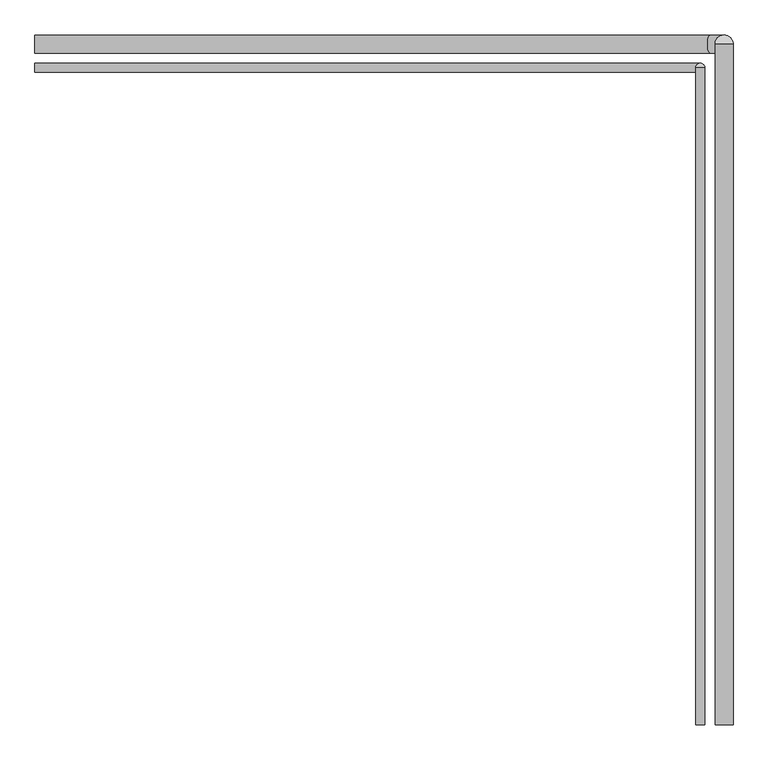
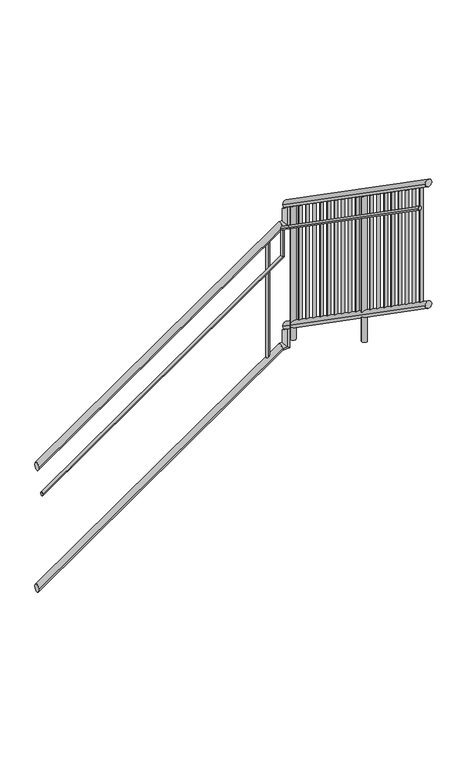
"""IFC4 building model written with IfcOpenShell, lengths in millimetres: railing geometry."""

from ifc_helpers import new_model, si_unit, frame, origin, place, context, project, spatial, circle_curve, ellipse_curve, source, transform, mapped, element, save
from ifc_brep_helpers import plane_surface, cylinder_surface, advanced_brep


def railing_cb7ceb08(model_context):
    return source(origin(), model_context, "Body", "AdvancedBrep", [
        advanced_brep(
        [(679.725551, -1750.2965465, 1656.5760546), (679.725551, -1801.0965465, 1656.5760546), (2577.6800324, -1750.2965465, 2974.6), (2577.6800324, -1801.0965465, 2974.6), (2617.625551, -1750.2965465, 2974.6), (2617.625551, -1801.0965465, 2974.6), (2617.625551, -1750.2965465, 3090.3743314), (2617.625551, -1801.0965465, 3125.6521091)],
        [
            (0, 1, ellipse_curve(frame((679.725551, -1775.6965465, 1656.5760546), z_axis=(-1.0, 0.0, 0.0), x_axis=(0.0, 0.0, -0.9999999999999999)), 30.9239454, 25.4)),
            (1, 0, ellipse_curve(frame((679.725551, -1775.6965465, 1656.5760546), z_axis=(-1.0, 0.0, 0.0), x_axis=(0.0, 0.0, -0.9999999999999999)), 30.9239454, 25.4)),
            (0, 2),
            (2, 3, ellipse_curve(frame((2577.6800324, -1775.6965465, 2974.6), z_axis=(-0.9542981624401503, 0.0, -0.2988561814039527), x_axis=(0.2988561814039518, 0.0, -0.9542981624401508)), 26.6164193, 25.4)),
            (3, 1),
            (3, 2, ellipse_curve(frame((2577.6800324, -1775.6965465, 2974.6), z_axis=(-0.9542981624401503, 0.0, -0.2988561814039527), x_axis=(0.2988561814039518, 0.0, -0.9542981624401508)), 26.6164193, 25.4)),
            (2, 4),
            (4, 5, ellipse_curve(frame((2617.625551, -1775.6965465, 2974.6), z_axis=(-0.7071067811865474, 0.0, -0.7071067811865476), x_axis=(-0.7071067811865478, 0.0, 0.7071067811865472)), 35.9210245, 25.4)),
            (5, 3),
            (5, 4, ellipse_curve(frame((2617.625551, -1775.6965465, 2974.6), z_axis=(-0.7071067811865474, 0.0, -0.7071067811865476), x_axis=(-0.7071067811865478, 0.0, 0.7071067811865472)), 35.9210245, 25.4)),
            (6, 7, ellipse_curve(frame((2617.625551, -1775.6965465, 3108.0132202), z_axis=(0.0, 0.5703958094953442, 0.8213699656732958), x_axis=(0.0, 0.8213699656732958, -0.5703958094953442)), 30.9239454, 25.4)),
            (7, 6, ellipse_curve(frame((2617.625551, -1775.6965465, 3108.0132202), z_axis=(0.0, 0.5703958094953442, 0.8213699656732958), x_axis=(0.0, 0.8213699656732958, -0.5703958094953442)), 30.9239454, 25.4)),
            (4, 6),
            (7, 5),
        ],
        [
            plane_surface(frame((679.725551, -1775.6965465, 1687.5), z_axis=(-1.0, 0.0, 0.0), x_axis=(0.0, 1.0, 0.0))),
            cylinder_surface(frame((694.2136045, -1775.6965465, 1666.6372029), z_axis=(-0.8213699656732956, 0.0, -0.5703958094953446), x_axis=(0.0, -1.0, 0.0)), 25.4),
            cylinder_surface(frame((2569.725551, -1775.6965465, 2974.6), z_axis=(-1.0, 0.0, 0.0), x_axis=(0.0, -1.0, 0.0)), 25.4),
            plane_surface(frame((2592.225551, -1775.6965465, 3108.0132202), z_axis=(0.0, 0.5703958094953442, 0.8213699656732958), x_axis=(1.0, 0.0, 0.0))),
            cylinder_surface(frame((2617.625551, -1775.6965465, 3000.0), z_axis=(0.0, 0.0, -1.0), x_axis=(0.0, -1.0, 0.0)), 25.4),
        ],
        [
            (0, [[1, 2]]),
            (1, [[-1, 3, 4, 5]]),
            (1, [[-2, -5, 6, -3]]),
            (2, [[-4, 7, 8, 9]]),
            (2, [[-6, -9, 10, -7]]),
            (3, [[11, 12]]),
            (4, [[-8, 13, -12, 14]]),
            (4, [[-10, -14, -11, -13]]),
        ],
    ),
        advanced_brep(
        [(2643.025551, -1775.6965465, 3138.9371657), (2592.225551, -1775.6965465, 3138.9371657), (2643.025551, -3691.0965465, 4469.0760546), (2592.225551, -3691.0965465, 4469.0760546)],
        [
            (0, 1, ellipse_curve(frame((2617.625551, -1775.6965465, 3138.9371657), z_axis=(0.0, 1.0, 0.0), x_axis=(0.0, 0.0, -1.0)), 30.9239454, 25.4)),
            (1, 0, ellipse_curve(frame((2617.625551, -1775.6965465, 3138.9371657), z_axis=(0.0, 1.0, 0.0), x_axis=(0.0, 0.0, -1.0)), 30.9239454, 25.4)),
            (2, 3, ellipse_curve(frame((2617.625551, -3691.0965465, 4469.0760546), z_axis=(0.0, -1.0, 0.0), x_axis=(0.0, 0.0, -1.0)), 30.9239454, 25.4)),
            (3, 2, ellipse_curve(frame((2617.625551, -3691.0965465, 4469.0760546), z_axis=(0.0, -1.0, 0.0), x_axis=(0.0, 0.0, -1.0)), 30.9239454, 25.4)),
            (0, 2),
            (3, 1),
        ],
        [
            plane_surface(frame((2617.625551, -1775.6965465, 3169.8611111), z_axis=(0.0, 1.0, 0.0), x_axis=(0.0, 0.0, -1.0))),
            plane_surface(frame((2617.625551, -3691.0965465, 4500.0), z_axis=(0.0, -1.0, 0.0), x_axis=(0.0, 0.0, -1.0))),
            cylinder_surface(frame((2617.625551, -1790.1846001, 3148.998314), z_axis=(0.0, 0.8213699656732958, -0.5703958094953442), x_axis=(-1.0, 0.0, 0.0)), 25.4),
        ],
        [
            (0, [[1, 2]]),
            (1, [[3, 4]]),
            (2, [[-1, 5, -4, 6]]),
            (2, [[-2, -6, -3, -5]]),
        ],
    ),
        advanced_brep(
        [(679.725551, -1829.9965465, 1472.0380273), (679.725551, -1855.3965465, 1472.0380273), (2550.625551, -1829.9965465, 2771.2741384), (2550.625551, -1855.3965465, 2771.2741384), (2550.625551, -1829.9965465, 2976.645499), (2550.625551, -1855.3965465, 2994.2843879)],
        [
            (0, 1, ellipse_curve(frame((679.725551, -1842.6965465, 1472.0380273), z_axis=(-1.0, 0.0, 0.0), x_axis=(0.0, 0.0, -1.0)), 15.4619727, 12.7)),
            (1, 0, ellipse_curve(frame((679.725551, -1842.6965465, 1472.0380273), z_axis=(-1.0, 0.0, 0.0), x_axis=(0.0, 0.0, -1.0)), 15.4619727, 12.7)),
            (0, 2),
            (2, 3, ellipse_curve(frame((2550.625551, -1842.6965465, 2771.2741384), z_axis=(-0.4634674694650399, 0.0, -0.8861139344055438), x_axis=(-0.8861139344055436, 0.0, 0.46346746946504)), 14.3322427, 12.7)),
            (3, 1),
            (3, 2, ellipse_curve(frame((2550.625551, -1842.6965465, 2771.2741384), z_axis=(-0.4634674694650399, 0.0, -0.8861139344055438), x_axis=(-0.8861139344055436, 0.0, 0.46346746946504)), 14.3322427, 12.7)),
            (4, 5, ellipse_curve(frame((2550.625551, -1842.6965465, 2985.4649435), z_axis=(0.0, 0.5703958094953442, 0.8213699656732959), x_axis=(0.0, 0.821369965673296, -0.5703958094953439)), 15.4619727, 12.7)),
            (5, 4, ellipse_curve(frame((2550.625551, -1842.6965465, 2985.4649435), z_axis=(0.0, 0.5703958094953442, 0.8213699656732959), x_axis=(0.0, 0.821369965673296, -0.5703958094953439)), 15.4619727, 12.7)),
            (2, 4),
            (5, 3),
        ],
        [
            plane_surface(frame((679.725551, -1842.6965465, 1487.5), z_axis=(-1.0, 0.0, 0.0), x_axis=(0.0, 1.0, 0.0))),
            cylinder_surface(frame((686.9695777, -1842.6965465, 1477.0686014), z_axis=(-0.8213699656732956, 0.0, -0.5703958094953444), x_axis=(0.0, -1.0, 0.0)), 12.7),
            plane_surface(frame((2537.925551, -1842.6965465, 2985.4649435), z_axis=(0.0, 0.5703958094953442, 0.8213699656732959), x_axis=(1.0, 0.0, 0.0))),
            cylinder_surface(frame((2550.625551, -1842.6965465, 2777.9166667), z_axis=(0.0, 0.0, -1.0), x_axis=(0.0, -1.0, 0.0)), 12.7),
        ],
        [
            (0, [[1, 2]]),
            (1, [[-1, 3, 4, 5]]),
            (1, [[-2, -5, 6, -3]]),
            (2, [[7, 8]]),
            (3, [[-4, 9, -8, 10]]),
            (3, [[-6, -10, -7, -9]]),
        ],
    ),
        advanced_brep(
        [(2563.325551, -1842.6965465, 3000.9269162), (2537.925551, -1842.6965465, 3000.9269162), (2563.325551, -3691.0965465, 4284.5380273), (2537.925551, -3691.0965465, 4284.5380273)],
        [
            (0, 1, ellipse_curve(frame((2550.625551, -1842.6965465, 3000.9269162), z_axis=(0.0, 1.0, 0.0), x_axis=(0.0, 0.0, -1.0)), 15.4619727, 12.7)),
            (1, 0, ellipse_curve(frame((2550.625551, -1842.6965465, 3000.9269162), z_axis=(0.0, 1.0, 0.0), x_axis=(0.0, 0.0, -1.0)), 15.4619727, 12.7)),
            (2, 3, ellipse_curve(frame((2550.625551, -3691.0965465, 4284.5380273), z_axis=(0.0, -1.0, 0.0), x_axis=(0.0, 0.0, -1.0)), 15.4619727, 12.7)),
            (3, 2, ellipse_curve(frame((2550.625551, -3691.0965465, 4284.5380273), z_axis=(0.0, -1.0, 0.0), x_axis=(0.0, 0.0, -1.0)), 15.4619727, 12.7)),
            (0, 2),
            (3, 1),
        ],
        [
            plane_surface(frame((2550.625551, -1842.6965465, 3016.3888889), z_axis=(0.0, 1.0, 0.0), x_axis=(0.0, 0.0, -1.0))),
            plane_surface(frame((2550.625551, -3691.0965465, 4300.0), z_axis=(0.0, -1.0, 0.0), x_axis=(0.0, 0.0, -1.0))),
            cylinder_surface(frame((2550.625551, -1849.9405733, 3005.9574903), z_axis=(0.0, 0.8213699656732959, -0.5703958094953442), x_axis=(-1.0, 0.0, 0.0)), 12.7),
        ],
        [
            (0, [[1, 2]]),
            (1, [[3, 4]]),
            (2, [[-1, 5, -4, 6]]),
            (2, [[-2, -6, -3, -5]]),
        ],
    ),
        advanced_brep(
        [(679.725551, -1750.2965465, 656.5760546), (679.725551, -1801.0965465, 656.5760546), (2577.6800324, -1750.2965465, 1974.6), (2577.6800324, -1801.0965465, 1974.6), (2617.625551, -1750.2965465, 1974.6), (2617.625551, -1801.0965465, 1974.6), (2617.625551, -1750.2965465, 2090.3743314), (2617.625551, -1801.0965465, 2125.6521091)],
        [
            (0, 1, ellipse_curve(frame((679.725551, -1775.6965465, 656.5760546), z_axis=(-1.0, 0.0, 0.0), x_axis=(0.0, 0.0, -1.0)), 30.9239454, 25.4)),
            (1, 0, ellipse_curve(frame((679.725551, -1775.6965465, 656.5760546), z_axis=(-1.0, 0.0, 0.0), x_axis=(0.0, 0.0, -1.0)), 30.9239454, 25.4)),
            (0, 2),
            (2, 3, ellipse_curve(frame((2577.6800324, -1775.6965465, 1974.6), z_axis=(-0.9542981624401505, 0.0, -0.29885618140395265), x_axis=(0.2988561814039529, 0.0, -0.9542981624401503)), 26.6164193, 25.4)),
            (3, 1),
            (3, 2, ellipse_curve(frame((2577.6800324, -1775.6965465, 1974.6), z_axis=(-0.9542981624401505, 0.0, -0.29885618140395265), x_axis=(0.2988561814039529, 0.0, -0.9542981624401503)), 26.6164193, 25.4)),
            (2, 4),
            (4, 5, ellipse_curve(frame((2617.625551, -1775.6965465, 1974.6), z_axis=(-0.7071067811865475, 0.0, -0.7071067811865475), x_axis=(-0.7071067811865476, 0.0, 0.7071067811865474)), 35.9210245, 25.4)),
            (5, 3),
            (5, 4, ellipse_curve(frame((2617.625551, -1775.6965465, 1974.6), z_axis=(-0.7071067811865475, 0.0, -0.7071067811865475), x_axis=(-0.7071067811865476, 0.0, 0.7071067811865474)), 35.9210245, 25.4)),
            (6, 7, ellipse_curve(frame((2617.625551, -1775.6965465, 2108.0132202), z_axis=(0.0, 0.5703958094953442, 0.8213699656732958), x_axis=(0.0, 0.8213699656732958, -0.5703958094953442)), 30.9239454, 25.4)),
            (7, 6, ellipse_curve(frame((2617.625551, -1775.6965465, 2108.0132202), z_axis=(0.0, 0.5703958094953442, 0.8213699656732958), x_axis=(0.0, 0.8213699656732958, -0.5703958094953442)), 30.9239454, 25.4)),
            (4, 6),
            (7, 5),
        ],
        [
            plane_surface(frame((679.725551, -1775.6965465, 687.5), z_axis=(-1.0, 0.0, 0.0), x_axis=(0.0, 1.0, 0.0))),
            cylinder_surface(frame((694.2136045, -1775.6965465, 666.6372029), z_axis=(-0.8213699656732956, 0.0, -0.5703958094953445), x_axis=(0.0, -1.0, 0.0)), 25.4),
            cylinder_surface(frame((2569.725551, -1775.6965465, 1974.6), z_axis=(-1.0, 0.0, 0.0), x_axis=(0.0, -1.0, 0.0)), 25.4),
            plane_surface(frame((2592.225551, -1775.6965465, 2108.0132202), z_axis=(0.0, 0.5703958094953442, 0.8213699656732958), x_axis=(1.0, 0.0, 0.0))),
            cylinder_surface(frame((2617.625551, -1775.6965465, 2000.0), z_axis=(0.0, 0.0, -1.0), x_axis=(0.0, -1.0, 0.0)), 25.4),
        ],
        [
            (0, [[1, 2]]),
            (1, [[-1, 3, 4, 5]]),
            (1, [[-2, -5, 6, -3]]),
            (2, [[-4, 7, 8, 9]]),
            (2, [[-6, -9, 10, -7]]),
            (3, [[11, 12]]),
            (4, [[-8, 13, -12, 14]]),
            (4, [[-10, -14, -11, -13]]),
        ],
    ),
        advanced_brep(
        [(2643.025551, -1775.6965465, 2138.9371657), (2592.225551, -1775.6965465, 2138.9371657), (2643.025551, -3691.0965465, 3469.0760546), (2592.225551, -3691.0965465, 3469.0760546)],
        [
            (0, 1, ellipse_curve(frame((2617.625551, -1775.6965465, 2138.9371657), z_axis=(0.0, 1.0, 0.0), x_axis=(0.0, 0.0, -1.0)), 30.9239454, 25.4)),
            (1, 0, ellipse_curve(frame((2617.625551, -1775.6965465, 2138.9371657), z_axis=(0.0, 1.0, 0.0), x_axis=(0.0, 0.0, -1.0)), 30.9239454, 25.4)),
            (2, 3, ellipse_curve(frame((2617.625551, -3691.0965465, 3469.0760546), z_axis=(0.0, -1.0, 0.0), x_axis=(0.0, 0.0, -1.0)), 30.9239454, 25.4)),
            (3, 2, ellipse_curve(frame((2617.625551, -3691.0965465, 3469.0760546), z_axis=(0.0, -1.0, 0.0), x_axis=(0.0, 0.0, -1.0)), 30.9239454, 25.4)),
            (0, 2),
            (3, 1),
        ],
        [
            plane_surface(frame((2617.625551, -1775.6965465, 2169.8611111), z_axis=(0.0, 1.0, 0.0), x_axis=(0.0, 0.0, -1.0))),
            plane_surface(frame((2617.625551, -3691.0965465, 3500.0), z_axis=(0.0, -1.0, 0.0), x_axis=(0.0, 0.0, -1.0))),
            cylinder_surface(frame((2617.625551, -1790.1846001, 2148.998314), z_axis=(0.0, 0.8213699656732958, -0.5703958094953442), x_axis=(-1.0, 0.0, 0.0)), 25.4),
        ],
        [
            (0, [[1, 2]]),
            (1, [[3, 4]]),
            (2, [[-1, 5, -4, 6]]),
            (2, [[-2, -6, -3, -5]]),
        ],
    ),
        advanced_brep(
        [(2605.125551, -3595.3265465, 4371.6451647), (2605.125551, -3595.3265465, 3433.4930556), (2630.125551, -3595.3265465, 3433.4930556), (2630.125551, -3595.3265465, 4371.6451647)],
        [
            (0, 1),
            (1, 2, ellipse_curve(frame((2617.625551, -3595.3265465, 3433.4930556), z_axis=(0.0, 0.5703958094953444, 0.8213699656732956), x_axis=(0.0, -0.8213699656732956, 0.5703958094953445)), 15.2184771, 12.5)),
            (2, 3),
            (3, 0, ellipse_curve(frame((2617.625551, -3595.3265465, 4371.6451647), z_axis=(0.0, -0.5703958094953457, -0.8213699656732947), x_axis=(0.0, -0.8213699656732947, 0.5703958094953456)), 15.2184771, 12.5)),
            (0, 3, ellipse_curve(frame((2617.625551, -3595.3265465, 4371.6451647), z_axis=(0.0, -0.5703958094953457, -0.8213699656732947), x_axis=(0.0, -0.8213699656732947, 0.5703958094953456)), 15.2184771, 12.5)),
            (2, 1, ellipse_curve(frame((2617.625551, -3595.3265465, 3433.4930556), z_axis=(0.0, 0.5703958094953444, 0.8213699656732956), x_axis=(0.0, -0.8213699656732956, 0.5703958094953445)), 15.2184771, 12.5)),
        ],
        [
            cylinder_surface(frame((2617.625551, -3595.3265465, 3333.4930556), z_axis=(0.0, 0.0, 1.0), x_axis=(1.0, 0.0, 0.0)), 12.5),
            plane_surface(frame((2642.625551, -3620.3265465, 4389.0062758), z_axis=(0.0, 0.5703958094953457, 0.8213699656732947), x_axis=(-1.0, 0.0, 0.0))),
            plane_surface(frame((2642.625551, -3570.3265465, 3416.1319444), z_axis=(0.0, -0.5703958094953444, -0.8213699656732956), x_axis=(-1.0, 0.0, 0.0))),
        ],
        [
            (0, [[1, 2, 3, 4]]),
            (0, [[-1, 5, -3, 6]]),
            (1, [[-4, -5]]),
            (2, [[-2, -6]]),
        ],
    ),
        advanced_brep(
        [(2605.125551, -3499.5565465, 4305.1382202), (2605.125551, -3499.5565465, 3366.9861111), (2630.125551, -3499.5565465, 3366.9861111), (2630.125551, -3499.5565465, 4305.1382202)],
        [
            (0, 1),
            (1, 2, ellipse_curve(frame((2617.625551, -3499.5565465, 3366.9861111), z_axis=(0.0, 0.5703958094953444, 0.8213699656732956), x_axis=(0.0, -0.8213699656732956, 0.5703958094953445)), 15.2184771, 12.5)),
            (2, 3),
            (3, 0, ellipse_curve(frame((2617.625551, -3499.5565465, 4305.1382202), z_axis=(0.0, -0.5703958094953457, -0.8213699656732947), x_axis=(0.0, -0.8213699656732947, 0.5703958094953456)), 15.2184771, 12.5)),
            (0, 3, ellipse_curve(frame((2617.625551, -3499.5565465, 4305.1382202), z_axis=(0.0, -0.5703958094953457, -0.8213699656732947), x_axis=(0.0, -0.8213699656732947, 0.5703958094953456)), 15.2184771, 12.5)),
            (2, 1, ellipse_curve(frame((2617.625551, -3499.5565465, 3366.9861111), z_axis=(0.0, 0.5703958094953444, 0.8213699656732956), x_axis=(0.0, -0.8213699656732956, 0.5703958094953445)), 15.2184771, 12.5)),
        ],
        [
            cylinder_surface(frame((2617.625551, -3499.5565465, 3266.9861111), z_axis=(0.0, 0.0, 1.0), x_axis=(1.0, 0.0, 0.0)), 12.5),
            plane_surface(frame((2642.625551, -3524.5565465, 4322.4993314), z_axis=(0.0, 0.5703958094953457, 0.8213699656732947), x_axis=(-1.0, 0.0, 0.0))),
            plane_surface(frame((2642.625551, -3474.5565465, 3349.625), z_axis=(0.0, -0.5703958094953444, -0.8213699656732956), x_axis=(-1.0, 0.0, 0.0))),
        ],
        [
            (0, [[1, 2, 3, 4]]),
            (0, [[-1, 5, -3, 6]]),
            (1, [[-4, -5]]),
            (2, [[-2, -6]]),
        ],
    ),
        advanced_brep(
        [(2605.125551, -3403.7865465, 4238.6312758), (2605.125551, -3403.7865465, 3300.4791667), (2630.125551, -3403.7865465, 3300.4791667), (2630.125551, -3403.7865465, 4238.6312758)],
        [
            (0, 1),
            (1, 2, ellipse_curve(frame((2617.625551, -3403.7865465, 3300.4791667), z_axis=(0.0, 0.5703958094953444, 0.8213699656732956), x_axis=(0.0, -0.8213699656732956, 0.5703958094953445)), 15.2184771, 12.5)),
            (2, 3),
            (3, 0, ellipse_curve(frame((2617.625551, -3403.7865465, 4238.6312758), z_axis=(0.0, -0.5703958094953457, -0.8213699656732947), x_axis=(0.0, -0.8213699656732947, 0.5703958094953456)), 15.2184771, 12.5)),
            (0, 3, ellipse_curve(frame((2617.625551, -3403.7865465, 4238.6312758), z_axis=(0.0, -0.5703958094953457, -0.8213699656732947), x_axis=(0.0, -0.8213699656732947, 0.5703958094953456)), 15.2184771, 12.5)),
            (2, 1, ellipse_curve(frame((2617.625551, -3403.7865465, 3300.4791667), z_axis=(0.0, 0.5703958094953444, 0.8213699656732956), x_axis=(0.0, -0.8213699656732956, 0.5703958094953445)), 15.2184771, 12.5)),
        ],
        [
            cylinder_surface(frame((2617.625551, -3403.7865465, 3200.4791667), z_axis=(0.0, 0.0, 1.0), x_axis=(1.0, 0.0, 0.0)), 12.5),
            plane_surface(frame((2642.625551, -3428.7865465, 4255.9923869), z_axis=(0.0, 0.5703958094953457, 0.8213699656732947), x_axis=(-1.0, 0.0, 0.0))),
            plane_surface(frame((2642.625551, -3378.7865465, 3283.1180556), z_axis=(0.0, -0.5703958094953444, -0.8213699656732956), x_axis=(-1.0, 0.0, 0.0))),
        ],
        [
            (0, [[1, 2, 3, 4]]),
            (0, [[-1, 5, -3, 6]]),
            (1, [[-4, -5]]),
            (2, [[-2, -6]]),
        ],
    ),
        advanced_brep(
        [(2605.125551, -3308.0165465, 4172.1243314), (2605.125551, -3308.0165465, 3233.9722222), (2630.125551, -3308.0165465, 3233.9722222), (2630.125551, -3308.0165465, 4172.1243314)],
        [
            (0, 1),
            (1, 2, ellipse_curve(frame((2617.625551, -3308.0165465, 3233.9722222), z_axis=(0.0, 0.5703958094953444, 0.8213699656732956), x_axis=(0.0, -0.8213699656732956, 0.5703958094953445)), 15.2184771, 12.5)),
            (2, 3),
            (3, 0, ellipse_curve(frame((2617.625551, -3308.0165465, 4172.1243314), z_axis=(0.0, -0.5703958094953457, -0.8213699656732947), x_axis=(0.0, -0.8213699656732947, 0.5703958094953456)), 15.2184771, 12.5)),
            (0, 3, ellipse_curve(frame((2617.625551, -3308.0165465, 4172.1243314), z_axis=(0.0, -0.5703958094953457, -0.8213699656732947), x_axis=(0.0, -0.8213699656732947, 0.5703958094953456)), 15.2184771, 12.5)),
            (2, 1, ellipse_curve(frame((2617.625551, -3308.0165465, 3233.9722222), z_axis=(0.0, 0.5703958094953444, 0.8213699656732956), x_axis=(0.0, -0.8213699656732956, 0.5703958094953445)), 15.2184771, 12.5)),
        ],
        [
            cylinder_surface(frame((2617.625551, -3308.0165465, 3133.9722222), z_axis=(0.0, 0.0, 1.0), x_axis=(1.0, 0.0, 0.0)), 12.5),
            plane_surface(frame((2642.625551, -3333.0165465, 4189.4854425), z_axis=(0.0, 0.5703958094953457, 0.8213699656732947), x_axis=(-1.0, 0.0, 0.0))),
            plane_surface(frame((2642.625551, -3283.0165465, 3216.6111111), z_axis=(0.0, -0.5703958094953444, -0.8213699656732956), x_axis=(-1.0, 0.0, 0.0))),
        ],
        [
            (0, [[1, 2, 3, 4]]),
            (0, [[-1, 5, -3, 6]]),
            (1, [[-4, -5]]),
            (2, [[-2, -6]]),
        ],
    ),
        advanced_brep(
        [(2605.125551, -3212.2465465, 4105.6173869), (2605.125551, -3212.2465465, 3167.4652778), (2630.125551, -3212.2465465, 3167.4652778), (2630.125551, -3212.2465465, 4105.6173869)],
        [
            (0, 1),
            (1, 2, ellipse_curve(frame((2617.625551, -3212.2465465, 3167.4652778), z_axis=(0.0, 0.5703958094953444, 0.8213699656732956), x_axis=(0.0, -0.8213699656732956, 0.5703958094953445)), 15.2184771, 12.5)),
            (2, 3),
            (3, 0, ellipse_curve(frame((2617.625551, -3212.2465465, 4105.6173869), z_axis=(0.0, -0.5703958094953457, -0.8213699656732947), x_axis=(0.0, -0.8213699656732947, 0.5703958094953456)), 15.2184771, 12.5)),
            (0, 3, ellipse_curve(frame((2617.625551, -3212.2465465, 4105.6173869), z_axis=(0.0, -0.5703958094953457, -0.8213699656732947), x_axis=(0.0, -0.8213699656732947, 0.5703958094953456)), 15.2184771, 12.5)),
            (2, 1, ellipse_curve(frame((2617.625551, -3212.2465465, 3167.4652778), z_axis=(0.0, 0.5703958094953444, 0.8213699656732956), x_axis=(0.0, -0.8213699656732956, 0.5703958094953445)), 15.2184771, 12.5)),
        ],
        [
            cylinder_surface(frame((2617.625551, -3212.2465465, 3067.4652778), z_axis=(0.0, 0.0, 1.0), x_axis=(1.0, 0.0, 0.0)), 12.5),
            plane_surface(frame((2642.625551, -3237.2465465, 4122.978498), z_axis=(0.0, 0.5703958094953457, 0.8213699656732947), x_axis=(-1.0, 0.0, 0.0))),
            plane_surface(frame((2642.625551, -3187.2465465, 3150.1041667), z_axis=(0.0, -0.5703958094953444, -0.8213699656732956), x_axis=(-1.0, 0.0, 0.0))),
        ],
        [
            (0, [[1, 2, 3, 4]]),
            (0, [[-1, 5, -3, 6]]),
            (1, [[-4, -5]]),
            (2, [[-2, -6]]),
        ],
    ),
        advanced_brep(
        [(2605.125551, -3116.4765465, 4039.1104425), (2605.125551, -3116.4765465, 3100.9583333), (2630.125551, -3116.4765465, 3100.9583333), (2630.125551, -3116.4765465, 4039.1104425)],
        [
            (0, 1),
            (1, 2, ellipse_curve(frame((2617.625551, -3116.4765465, 3100.9583333), z_axis=(0.0, 0.5703958094953444, 0.8213699656732956), x_axis=(0.0, -0.8213699656732956, 0.5703958094953445)), 15.2184771, 12.5)),
            (2, 3),
            (3, 0, ellipse_curve(frame((2617.625551, -3116.4765465, 4039.1104425), z_axis=(0.0, -0.5703958094953457, -0.8213699656732947), x_axis=(0.0, -0.8213699656732947, 0.5703958094953456)), 15.2184771, 12.5)),
            (0, 3, ellipse_curve(frame((2617.625551, -3116.4765465, 4039.1104425), z_axis=(0.0, -0.5703958094953457, -0.8213699656732947), x_axis=(0.0, -0.8213699656732947, 0.5703958094953456)), 15.2184771, 12.5)),
            (2, 1, ellipse_curve(frame((2617.625551, -3116.4765465, 3100.9583333), z_axis=(0.0, 0.5703958094953444, 0.8213699656732956), x_axis=(0.0, -0.8213699656732956, 0.5703958094953445)), 15.2184771, 12.5)),
        ],
        [
            cylinder_surface(frame((2617.625551, -3116.4765465, 3000.9583333), z_axis=(0.0, 0.0, 1.0), x_axis=(1.0, 0.0, 0.0)), 12.5),
            plane_surface(frame((2642.625551, -3141.4765465, 4056.4715536), z_axis=(0.0, 0.5703958094953457, 0.8213699656732947), x_axis=(-1.0, 0.0, 0.0))),
            plane_surface(frame((2642.625551, -3091.4765465, 3083.5972222), z_axis=(0.0, -0.5703958094953444, -0.8213699656732956), x_axis=(-1.0, 0.0, 0.0))),
        ],
        [
            (0, [[1, 2, 3, 4]]),
            (0, [[-1, 5, -3, 6]]),
            (1, [[-4, -5]]),
            (2, [[-2, -6]]),
        ],
    ),
        advanced_brep(
        [(2605.125551, -3020.7065465, 3972.603498), (2605.125551, -3020.7065465, 3034.4513889), (2630.125551, -3020.7065465, 3034.4513889), (2630.125551, -3020.7065465, 3972.603498)],
        [
            (0, 1),
            (1, 2, ellipse_curve(frame((2617.625551, -3020.7065465, 3034.4513889), z_axis=(0.0, 0.5703958094953444, 0.8213699656732956), x_axis=(0.0, -0.8213699656732956, 0.5703958094953445)), 15.2184771, 12.5)),
            (2, 3),
            (3, 0, ellipse_curve(frame((2617.625551, -3020.7065465, 3972.603498), z_axis=(0.0, -0.5703958094953457, -0.8213699656732947), x_axis=(0.0, -0.8213699656732947, 0.5703958094953456)), 15.2184771, 12.5)),
            (0, 3, ellipse_curve(frame((2617.625551, -3020.7065465, 3972.603498), z_axis=(0.0, -0.5703958094953457, -0.8213699656732947), x_axis=(0.0, -0.8213699656732947, 0.5703958094953456)), 15.2184771, 12.5)),
            (2, 1, ellipse_curve(frame((2617.625551, -3020.7065465, 3034.4513889), z_axis=(0.0, 0.5703958094953444, 0.8213699656732956), x_axis=(0.0, -0.8213699656732956, 0.5703958094953445)), 15.2184771, 12.5)),
        ],
        [
            cylinder_surface(frame((2617.625551, -3020.7065465, 2934.4513889), z_axis=(0.0, 0.0, 1.0), x_axis=(1.0, 0.0, 0.0)), 12.5),
            plane_surface(frame((2642.625551, -3045.7065465, 3989.9646091), z_axis=(0.0, 0.5703958094953457, 0.8213699656732947), x_axis=(-1.0, 0.0, 0.0))),
            plane_surface(frame((2642.625551, -2995.7065465, 3017.0902778), z_axis=(0.0, -0.5703958094953444, -0.8213699656732956), x_axis=(-1.0, 0.0, 0.0))),
        ],
        [
            (0, [[1, 2, 3, 4]]),
            (0, [[-1, 5, -3, 6]]),
            (1, [[-4, -5]]),
            (2, [[-2, -6]]),
        ],
    ),
        advanced_brep(
        [(2605.125551, -2924.9365465, 3906.0965536), (2605.125551, -2924.9365465, 2967.9444444), (2630.125551, -2924.9365465, 2967.9444444), (2630.125551, -2924.9365465, 3906.0965536)],
        [
            (0, 1),
            (1, 2, ellipse_curve(frame((2617.625551, -2924.9365465, 2967.9444444), z_axis=(0.0, 0.5703958094953444, 0.8213699656732956), x_axis=(0.0, -0.8213699656732956, 0.5703958094953445)), 15.2184771, 12.5)),
            (2, 3),
            (3, 0, ellipse_curve(frame((2617.625551, -2924.9365465, 3906.0965536), z_axis=(0.0, -0.5703958094953457, -0.8213699656732947), x_axis=(0.0, -0.8213699656732947, 0.5703958094953456)), 15.2184771, 12.5)),
            (0, 3, ellipse_curve(frame((2617.625551, -2924.9365465, 3906.0965536), z_axis=(0.0, -0.5703958094953457, -0.8213699656732947), x_axis=(0.0, -0.8213699656732947, 0.5703958094953456)), 15.2184771, 12.5)),
            (2, 1, ellipse_curve(frame((2617.625551, -2924.9365465, 2967.9444444), z_axis=(0.0, 0.5703958094953444, 0.8213699656732956), x_axis=(0.0, -0.8213699656732956, 0.5703958094953445)), 15.2184771, 12.5)),
        ],
        [
            cylinder_surface(frame((2617.625551, -2924.9365465, 2867.9444444), z_axis=(0.0, 0.0, 1.0), x_axis=(1.0, 0.0, 0.0)), 12.5),
            plane_surface(frame((2642.625551, -2949.9365465, 3923.4576647), z_axis=(0.0, 0.5703958094953457, 0.8213699656732947), x_axis=(-1.0, 0.0, 0.0))),
            plane_surface(frame((2642.625551, -2899.9365465, 2950.5833333), z_axis=(0.0, -0.5703958094953444, -0.8213699656732956), x_axis=(-1.0, 0.0, 0.0))),
        ],
        [
            (0, [[1, 2, 3, 4]]),
            (0, [[-1, 5, -3, 6]]),
            (1, [[-4, -5]]),
            (2, [[-2, -6]]),
        ],
    ),
        advanced_brep(
        [(2596.625551, -2829.1665465, 3839.5896091), (2596.625551, -2829.1665465, 2650.0), (2638.625551, -2829.1665465, 2650.0), (2638.625551, -2829.1665465, 3839.5896091)],
        [
            (0, 1),
            (1, 2, circle_curve(frame((2617.625551, -2829.1665465, 2650.0), z_axis=(0.0, 0.0, 1.0), x_axis=(1.0, 0.0, 0.0)), 21.0)),
            (2, 3),
            (3, 0, ellipse_curve(frame((2617.625551, -2829.1665465, 3839.5896091), z_axis=(0.0, -0.5703958094953442, -0.8213699656732958), x_axis=(0.0, -0.8213699656732958, 0.5703958094953442)), 25.5670415, 21.0)),
            (0, 3, ellipse_curve(frame((2617.625551, -2829.1665465, 3839.5896091), z_axis=(0.0, -0.5703958094953442, -0.8213699656732958), x_axis=(0.0, -0.8213699656732958, 0.5703958094953442)), 25.5670415, 21.0)),
            (2, 1, circle_curve(frame((2617.625551, -2829.1665465, 2650.0), z_axis=(0.0, 0.0, 1.0), x_axis=(1.0, 0.0, 0.0)), 21.0)),
        ],
        [
            cylinder_surface(frame((2617.625551, -2829.1665465, 2550.0), z_axis=(0.0, 0.0, 1.0), x_axis=(1.0, 0.0, 0.0)), 21.0),
            plane_surface(frame((2659.625551, -2871.1665465, 3868.7562758), z_axis=(0.0, 0.5703958094953442, 0.8213699656732958), x_axis=(-1.0, 0.0, 0.0))),
            plane_surface(frame((2659.625551, -2787.1665465, 2650.0), z_axis=(0.0, 0.0, -1.0), x_axis=(-1.0, 0.0, 0.0))),
        ],
        [
            (0, [[1, 2, 3, 4]]),
            (0, [[-1, 5, -3, 6]]),
            (1, [[-4, -5]]),
            (2, [[-2, -6]]),
        ],
    ),
        advanced_brep(
        [(2605.125551, -2733.3965465, 3773.0826647), (2605.125551, -2733.3965465, 2834.9305556), (2630.125551, -2733.3965465, 2834.9305556), (2630.125551, -2733.3965465, 3773.0826647)],
        [
            (0, 1),
            (1, 2, ellipse_curve(frame((2617.625551, -2733.3965465, 2834.9305556), z_axis=(0.0, 0.5703958094953444, 0.8213699656732956), x_axis=(0.0, -0.8213699656732956, 0.5703958094953445)), 15.2184771, 12.5)),
            (2, 3),
            (3, 0, ellipse_curve(frame((2617.625551, -2733.3965465, 3773.0826647), z_axis=(0.0, -0.5703958094953457, -0.8213699656732947), x_axis=(0.0, -0.8213699656732947, 0.5703958094953456)), 15.2184771, 12.5)),
            (0, 3, ellipse_curve(frame((2617.625551, -2733.3965465, 3773.0826647), z_axis=(0.0, -0.5703958094953457, -0.8213699656732947), x_axis=(0.0, -0.8213699656732947, 0.5703958094953456)), 15.2184771, 12.5)),
            (2, 1, ellipse_curve(frame((2617.625551, -2733.3965465, 2834.9305556), z_axis=(0.0, 0.5703958094953444, 0.8213699656732956), x_axis=(0.0, -0.8213699656732956, 0.5703958094953445)), 15.2184771, 12.5)),
        ],
        [
            cylinder_surface(frame((2617.625551, -2733.3965465, 2734.9305556), z_axis=(0.0, 0.0, 1.0), x_axis=(1.0, 0.0, 0.0)), 12.5),
            plane_surface(frame((2642.625551, -2758.3965465, 3790.4437758), z_axis=(0.0, 0.5703958094953457, 0.8213699656732947), x_axis=(-1.0, 0.0, 0.0))),
            plane_surface(frame((2642.625551, -2708.3965465, 2817.5694444), z_axis=(0.0, -0.5703958094953444, -0.8213699656732956), x_axis=(-1.0, 0.0, 0.0))),
        ],
        [
            (0, [[1, 2, 3, 4]]),
            (0, [[-1, 5, -3, 6]]),
            (1, [[-4, -5]]),
            (2, [[-2, -6]]),
        ],
    ),
        advanced_brep(
        [(2605.125551, -2637.6265465, 3706.5757202), (2605.125551, -2637.6265465, 2768.4236111), (2630.125551, -2637.6265465, 2768.4236111), (2630.125551, -2637.6265465, 3706.5757202)],
        [
            (0, 1),
            (1, 2, ellipse_curve(frame((2617.625551, -2637.6265465, 2768.4236111), z_axis=(0.0, 0.5703958094953444, 0.8213699656732956), x_axis=(0.0, -0.8213699656732956, 0.5703958094953445)), 15.2184771, 12.5)),
            (2, 3),
            (3, 0, ellipse_curve(frame((2617.625551, -2637.6265465, 3706.5757202), z_axis=(0.0, -0.5703958094953457, -0.8213699656732947), x_axis=(0.0, -0.8213699656732947, 0.5703958094953456)), 15.2184771, 12.5)),
            (0, 3, ellipse_curve(frame((2617.625551, -2637.6265465, 3706.5757202), z_axis=(0.0, -0.5703958094953457, -0.8213699656732947), x_axis=(0.0, -0.8213699656732947, 0.5703958094953456)), 15.2184771, 12.5)),
            (2, 1, ellipse_curve(frame((2617.625551, -2637.6265465, 2768.4236111), z_axis=(0.0, 0.5703958094953444, 0.8213699656732956), x_axis=(0.0, -0.8213699656732956, 0.5703958094953445)), 15.2184771, 12.5)),
        ],
        [
            cylinder_surface(frame((2617.625551, -2637.6265465, 2668.4236111), z_axis=(0.0, 0.0, 1.0), x_axis=(1.0, 0.0, 0.0)), 12.5),
            plane_surface(frame((2642.625551, -2662.6265465, 3723.9368314), z_axis=(0.0, 0.5703958094953457, 0.8213699656732947), x_axis=(-1.0, 0.0, 0.0))),
            plane_surface(frame((2642.625551, -2612.6265465, 2751.0625), z_axis=(0.0, -0.5703958094953444, -0.8213699656732956), x_axis=(-1.0, 0.0, 0.0))),
        ],
        [
            (0, [[1, 2, 3, 4]]),
            (0, [[-1, 5, -3, 6]]),
            (1, [[-4, -5]]),
            (2, [[-2, -6]]),
        ],
    ),
        advanced_brep(
        [(2605.125551, -2541.8565465, 3640.0687758), (2605.125551, -2541.8565465, 2701.9166667), (2630.125551, -2541.8565465, 2701.9166667), (2630.125551, -2541.8565465, 3640.0687758)],
        [
            (0, 1),
            (1, 2, ellipse_curve(frame((2617.625551, -2541.8565465, 2701.9166667), z_axis=(0.0, 0.5703958094953444, 0.8213699656732956), x_axis=(0.0, -0.8213699656732956, 0.5703958094953445)), 15.2184771, 12.5)),
            (2, 3),
            (3, 0, ellipse_curve(frame((2617.625551, -2541.8565465, 3640.0687758), z_axis=(0.0, -0.5703958094953457, -0.8213699656732947), x_axis=(0.0, -0.8213699656732947, 0.5703958094953456)), 15.2184771, 12.5)),
            (0, 3, ellipse_curve(frame((2617.625551, -2541.8565465, 3640.0687758), z_axis=(0.0, -0.5703958094953457, -0.8213699656732947), x_axis=(0.0, -0.8213699656732947, 0.5703958094953456)), 15.2184771, 12.5)),
            (2, 1, ellipse_curve(frame((2617.625551, -2541.8565465, 2701.9166667), z_axis=(0.0, 0.5703958094953444, 0.8213699656732956), x_axis=(0.0, -0.8213699656732956, 0.5703958094953445)), 15.2184771, 12.5)),
        ],
        [
            cylinder_surface(frame((2617.625551, -2541.8565465, 2601.9166667), z_axis=(0.0, 0.0, 1.0), x_axis=(1.0, 0.0, 0.0)), 12.5),
            plane_surface(frame((2642.625551, -2566.8565465, 3657.4298869), z_axis=(0.0, 0.5703958094953457, 0.8213699656732947), x_axis=(-1.0, 0.0, 0.0))),
            plane_surface(frame((2642.625551, -2516.8565465, 2684.5555556), z_axis=(0.0, -0.5703958094953444, -0.8213699656732956), x_axis=(-1.0, 0.0, 0.0))),
        ],
        [
            (0, [[1, 2, 3, 4]]),
            (0, [[-1, 5, -3, 6]]),
            (1, [[-4, -5]]),
            (2, [[-2, -6]]),
        ],
    ),
        advanced_brep(
        [(2605.125551, -2446.0865465, 3573.5618314), (2605.125551, -2446.0865465, 2635.4097222), (2630.125551, -2446.0865465, 2635.4097222), (2630.125551, -2446.0865465, 3573.5618314)],
        [
            (0, 1),
            (1, 2, ellipse_curve(frame((2617.625551, -2446.0865465, 2635.4097222), z_axis=(0.0, 0.5703958094953444, 0.8213699656732956), x_axis=(0.0, -0.8213699656732956, 0.5703958094953445)), 15.2184771, 12.5)),
            (2, 3),
            (3, 0, ellipse_curve(frame((2617.625551, -2446.0865465, 3573.5618314), z_axis=(0.0, -0.5703958094953457, -0.8213699656732947), x_axis=(0.0, -0.8213699656732947, 0.5703958094953456)), 15.2184771, 12.5)),
            (0, 3, ellipse_curve(frame((2617.625551, -2446.0865465, 3573.5618314), z_axis=(0.0, -0.5703958094953457, -0.8213699656732947), x_axis=(0.0, -0.8213699656732947, 0.5703958094953456)), 15.2184771, 12.5)),
            (2, 1, ellipse_curve(frame((2617.625551, -2446.0865465, 2635.4097222), z_axis=(0.0, 0.5703958094953444, 0.8213699656732956), x_axis=(0.0, -0.8213699656732956, 0.5703958094953445)), 15.2184771, 12.5)),
        ],
        [
            cylinder_surface(frame((2617.625551, -2446.0865465, 2535.4097222), z_axis=(0.0, 0.0, 1.0), x_axis=(1.0, 0.0, 0.0)), 12.5),
            plane_surface(frame((2642.625551, -2471.0865465, 3590.9229425), z_axis=(0.0, 0.5703958094953457, 0.8213699656732947), x_axis=(-1.0, 0.0, 0.0))),
            plane_surface(frame((2642.625551, -2421.0865465, 2618.0486111), z_axis=(0.0, -0.5703958094953444, -0.8213699656732956), x_axis=(-1.0, 0.0, 0.0))),
        ],
        [
            (0, [[1, 2, 3, 4]]),
            (0, [[-1, 5, -3, 6]]),
            (1, [[-4, -5]]),
            (2, [[-2, -6]]),
        ],
    ),
        advanced_brep(
        [(2605.125551, -2350.3165465, 3507.0548869), (2605.125551, -2350.3165465, 2568.9027778), (2630.125551, -2350.3165465, 2568.9027778), (2630.125551, -2350.3165465, 3507.0548869)],
        [
            (0, 1),
            (1, 2, ellipse_curve(frame((2617.625551, -2350.3165465, 2568.9027778), z_axis=(0.0, 0.5703958094953444, 0.8213699656732956), x_axis=(0.0, -0.8213699656732956, 0.5703958094953445)), 15.2184771, 12.5)),
            (2, 3),
            (3, 0, ellipse_curve(frame((2617.625551, -2350.3165465, 3507.0548869), z_axis=(0.0, -0.5703958094953457, -0.8213699656732947), x_axis=(0.0, -0.8213699656732947, 0.5703958094953456)), 15.2184771, 12.5)),
            (0, 3, ellipse_curve(frame((2617.625551, -2350.3165465, 3507.0548869), z_axis=(0.0, -0.5703958094953457, -0.8213699656732947), x_axis=(0.0, -0.8213699656732947, 0.5703958094953456)), 15.2184771, 12.5)),
            (2, 1, ellipse_curve(frame((2617.625551, -2350.3165465, 2568.9027778), z_axis=(0.0, 0.5703958094953444, 0.8213699656732956), x_axis=(0.0, -0.8213699656732956, 0.5703958094953445)), 15.2184771, 12.5)),
        ],
        [
            cylinder_surface(frame((2617.625551, -2350.3165465, 2468.9027778), z_axis=(0.0, 0.0, 1.0), x_axis=(1.0, 0.0, 0.0)), 12.5),
            plane_surface(frame((2642.625551, -2375.3165465, 3524.415998), z_axis=(0.0, 0.5703958094953457, 0.8213699656732947), x_axis=(-1.0, 0.0, 0.0))),
            plane_surface(frame((2642.625551, -2325.3165465, 2551.5416667), z_axis=(0.0, -0.5703958094953444, -0.8213699656732956), x_axis=(-1.0, 0.0, 0.0))),
        ],
        [
            (0, [[1, 2, 3, 4]]),
            (0, [[-1, 5, -3, 6]]),
            (1, [[-4, -5]]),
            (2, [[-2, -6]]),
        ],
    ),
        advanced_brep(
        [(2605.125551, -2254.5465465, 3440.5479425), (2605.125551, -2254.5465465, 2502.3958333), (2630.125551, -2254.5465465, 2502.3958333), (2630.125551, -2254.5465465, 3440.5479425)],
        [
            (0, 1),
            (1, 2, ellipse_curve(frame((2617.625551, -2254.5465465, 2502.3958333), z_axis=(0.0, 0.5703958094953444, 0.8213699656732956), x_axis=(0.0, -0.8213699656732956, 0.5703958094953445)), 15.2184771, 12.5)),
            (2, 3),
            (3, 0, ellipse_curve(frame((2617.625551, -2254.5465465, 3440.5479425), z_axis=(0.0, -0.5703958094953457, -0.8213699656732947), x_axis=(0.0, -0.8213699656732947, 0.5703958094953456)), 15.2184771, 12.5)),
            (0, 3, ellipse_curve(frame((2617.625551, -2254.5465465, 3440.5479425), z_axis=(0.0, -0.5703958094953457, -0.8213699656732947), x_axis=(0.0, -0.8213699656732947, 0.5703958094953456)), 15.2184771, 12.5)),
            (2, 1, ellipse_curve(frame((2617.625551, -2254.5465465, 2502.3958333), z_axis=(0.0, 0.5703958094953444, 0.8213699656732956), x_axis=(0.0, -0.8213699656732956, 0.5703958094953445)), 15.2184771, 12.5)),
        ],
        [
            cylinder_surface(frame((2617.625551, -2254.5465465, 2402.3958333), z_axis=(0.0, 0.0, 1.0), x_axis=(1.0, 0.0, 0.0)), 12.5),
            plane_surface(frame((2642.625551, -2279.5465465, 3457.9090536), z_axis=(0.0, 0.5703958094953457, 0.8213699656732947), x_axis=(-1.0, 0.0, 0.0))),
            plane_surface(frame((2642.625551, -2229.5465465, 2485.0347222), z_axis=(0.0, -0.5703958094953444, -0.8213699656732956), x_axis=(-1.0, 0.0, 0.0))),
        ],
        [
            (0, [[1, 2, 3, 4]]),
            (0, [[-1, 5, -3, 6]]),
            (1, [[-4, -5]]),
            (2, [[-2, -6]]),
        ],
    ),
        advanced_brep(
        [(2605.125551, -2158.7765465, 3374.040998), (2605.125551, -2158.7765465, 2435.8888889), (2630.125551, -2158.7765465, 2435.8888889), (2630.125551, -2158.7765465, 3374.040998)],
        [
            (0, 1),
            (1, 2, ellipse_curve(frame((2617.625551, -2158.7765465, 2435.8888889), z_axis=(0.0, 0.5703958094953444, 0.8213699656732956), x_axis=(0.0, -0.8213699656732956, 0.5703958094953445)), 15.2184771, 12.5)),
            (2, 3),
            (3, 0, ellipse_curve(frame((2617.625551, -2158.7765465, 3374.040998), z_axis=(0.0, -0.5703958094953457, -0.8213699656732947), x_axis=(0.0, -0.8213699656732947, 0.5703958094953456)), 15.2184771, 12.5)),
            (0, 3, ellipse_curve(frame((2617.625551, -2158.7765465, 3374.040998), z_axis=(0.0, -0.5703958094953457, -0.8213699656732947), x_axis=(0.0, -0.8213699656732947, 0.5703958094953456)), 15.2184771, 12.5)),
            (2, 1, ellipse_curve(frame((2617.625551, -2158.7765465, 2435.8888889), z_axis=(0.0, 0.5703958094953444, 0.8213699656732956), x_axis=(0.0, -0.8213699656732956, 0.5703958094953445)), 15.2184771, 12.5)),
        ],
        [
            cylinder_surface(frame((2617.625551, -2158.7765465, 2335.8888889), z_axis=(0.0, 0.0, 1.0), x_axis=(1.0, 0.0, 0.0)), 12.5),
            plane_surface(frame((2642.625551, -2183.7765465, 3391.4021091), z_axis=(0.0, 0.5703958094953457, 0.8213699656732947), x_axis=(-1.0, 0.0, 0.0))),
            plane_surface(frame((2642.625551, -2133.7765465, 2418.5277778), z_axis=(0.0, -0.5703958094953444, -0.8213699656732956), x_axis=(-1.0, 0.0, 0.0))),
        ],
        [
            (0, [[1, 2, 3, 4]]),
            (0, [[-1, 5, -3, 6]]),
            (1, [[-4, -5]]),
            (2, [[-2, -6]]),
        ],
    ),
        advanced_brep(
        [(2605.125551, -2063.0065465, 3307.5340536), (2605.125551, -2063.0065465, 2369.3819444), (2630.125551, -2063.0065465, 2369.3819444), (2630.125551, -2063.0065465, 3307.5340536)],
        [
            (0, 1),
            (1, 2, ellipse_curve(frame((2617.625551, -2063.0065465, 2369.3819444), z_axis=(0.0, 0.5703958094953444, 0.8213699656732956), x_axis=(0.0, -0.8213699656732956, 0.5703958094953445)), 15.2184771, 12.5)),
            (2, 3),
            (3, 0, ellipse_curve(frame((2617.625551, -2063.0065465, 3307.5340536), z_axis=(0.0, -0.5703958094953457, -0.8213699656732947), x_axis=(0.0, -0.8213699656732947, 0.5703958094953456)), 15.2184771, 12.5)),
            (0, 3, ellipse_curve(frame((2617.625551, -2063.0065465, 3307.5340536), z_axis=(0.0, -0.5703958094953457, -0.8213699656732947), x_axis=(0.0, -0.8213699656732947, 0.5703958094953456)), 15.2184771, 12.5)),
            (2, 1, ellipse_curve(frame((2617.625551, -2063.0065465, 2369.3819444), z_axis=(0.0, 0.5703958094953444, 0.8213699656732956), x_axis=(0.0, -0.8213699656732956, 0.5703958094953445)), 15.2184771, 12.5)),
        ],
        [
            cylinder_surface(frame((2617.625551, -2063.0065465, 2269.3819444), z_axis=(0.0, 0.0, 1.0), x_axis=(1.0, 0.0, 0.0)), 12.5),
            plane_surface(frame((2642.625551, -2088.0065465, 3324.8951647), z_axis=(0.0, 0.5703958094953457, 0.8213699656732947), x_axis=(-1.0, 0.0, 0.0))),
            plane_surface(frame((2642.625551, -2038.0065465, 2352.0208333), z_axis=(0.0, -0.5703958094953444, -0.8213699656732956), x_axis=(-1.0, 0.0, 0.0))),
        ],
        [
            (0, [[1, 2, 3, 4]]),
            (0, [[-1, 5, -3, 6]]),
            (1, [[-4, -5]]),
            (2, [[-2, -6]]),
        ],
    ),
        advanced_brep(
        [(2605.125551, -1967.2365465, 3241.0271091), (2605.125551, -1967.2365465, 2302.875), (2630.125551, -1967.2365465, 2302.875), (2630.125551, -1967.2365465, 3241.0271091)],
        [
            (0, 1),
            (1, 2, ellipse_curve(frame((2617.625551, -1967.2365465, 2302.875), z_axis=(0.0, 0.5703958094953444, 0.8213699656732956), x_axis=(0.0, -0.8213699656732956, 0.5703958094953445)), 15.2184771, 12.5)),
            (2, 3),
            (3, 0, ellipse_curve(frame((2617.625551, -1967.2365465, 3241.0271091), z_axis=(0.0, -0.5703958094953457, -0.8213699656732947), x_axis=(0.0, -0.8213699656732947, 0.5703958094953456)), 15.2184771, 12.5)),
            (0, 3, ellipse_curve(frame((2617.625551, -1967.2365465, 3241.0271091), z_axis=(0.0, -0.5703958094953457, -0.8213699656732947), x_axis=(0.0, -0.8213699656732947, 0.5703958094953456)), 15.2184771, 12.5)),
            (2, 1, ellipse_curve(frame((2617.625551, -1967.2365465, 2302.875), z_axis=(0.0, 0.5703958094953444, 0.8213699656732956), x_axis=(0.0, -0.8213699656732956, 0.5703958094953445)), 15.2184771, 12.5)),
        ],
        [
            cylinder_surface(frame((2617.625551, -1967.2365465, 2202.875), z_axis=(0.0, 0.0, 1.0), x_axis=(1.0, 0.0, 0.0)), 12.5),
            plane_surface(frame((2642.625551, -1992.2365465, 3258.3882202), z_axis=(0.0, 0.5703958094953457, 0.8213699656732947), x_axis=(-1.0, 0.0, 0.0))),
            plane_surface(frame((2642.625551, -1942.2365465, 2285.5138889), z_axis=(0.0, -0.5703958094953444, -0.8213699656732956), x_axis=(-1.0, 0.0, 0.0))),
        ],
        [
            (0, [[1, 2, 3, 4]]),
            (0, [[-1, 5, -3, 6]]),
            (1, [[-4, -5]]),
            (2, [[-2, -6]]),
        ],
    ),
        advanced_brep(
        [(2596.625551, -1871.4665465, 3174.5201647), (2596.625551, -1871.4665465, 2087.5), (2638.625551, -1871.4665465, 2087.5), (2638.625551, -1871.4665465, 3174.5201647)],
        [
            (0, 1),
            (1, 2, circle_curve(frame((2617.625551, -1871.4665465, 2087.5), z_axis=(0.0, 0.0, 1.0), x_axis=(1.0, 0.0, 0.0)), 21.0)),
            (2, 3),
            (3, 0, ellipse_curve(frame((2617.625551, -1871.4665465, 3174.5201647), z_axis=(0.0, -0.5703958094953442, -0.8213699656732958), x_axis=(0.0, -0.8213699656732958, 0.5703958094953442)), 25.5670415, 21.0)),
            (0, 3, ellipse_curve(frame((2617.625551, -1871.4665465, 3174.5201647), z_axis=(0.0, -0.5703958094953442, -0.8213699656732958), x_axis=(0.0, -0.8213699656732958, 0.5703958094953442)), 25.5670415, 21.0)),
            (2, 1, circle_curve(frame((2617.625551, -1871.4665465, 2087.5), z_axis=(0.0, 0.0, 1.0), x_axis=(1.0, 0.0, 0.0)), 21.0)),
        ],
        [
            cylinder_surface(frame((2617.625551, -1871.4665465, 1987.5), z_axis=(0.0, 0.0, 1.0), x_axis=(1.0, 0.0, 0.0)), 21.0),
            plane_surface(frame((2659.625551, -1913.4665465, 3203.6868314), z_axis=(0.0, 0.5703958094953442, 0.8213699656732958), x_axis=(-1.0, 0.0, 0.0))),
            plane_surface(frame((2659.625551, -1829.4665465, 2087.5), z_axis=(0.0, 0.0, -1.0), x_axis=(-1.0, 0.0, 0.0))),
        ],
        [
            (0, [[1, 2, 3, 4]]),
            (0, [[-1, 5, -3, 6]]),
            (1, [[-4, -5]]),
            (2, [[-2, -6]]),
        ],
    ),
        advanced_brep(
        [(2475.225551, -1788.1965465, 2872.5271091), (2475.225551, -1788.1965465, 1934.375), (2475.225551, -1763.1965465, 1934.375), (2475.225551, -1763.1965465, 2872.5271091)],
        [
            (0, 1),
            (1, 2, ellipse_curve(frame((2475.225551, -1775.6965465, 1934.375), z_axis=(-0.5703958094953444, 0.0, 0.8213699656732956), x_axis=(0.8213699656732956, 0.0, 0.5703958094953445)), 15.2184771, 12.5)),
            (2, 3),
            (3, 0, ellipse_curve(frame((2475.225551, -1775.6965465, 2872.5271091), z_axis=(0.5703958094953457, 0.0, -0.8213699656732947), x_axis=(0.8213699656732947, 0.0, 0.5703958094953456)), 15.2184771, 12.5)),
            (0, 3, ellipse_curve(frame((2475.225551, -1775.6965465, 2872.5271091), z_axis=(0.5703958094953457, 0.0, -0.8213699656732947), x_axis=(0.8213699656732947, 0.0, 0.5703958094953456)), 15.2184771, 12.5)),
            (2, 1, ellipse_curve(frame((2475.225551, -1775.6965465, 1934.375), z_axis=(-0.5703958094953444, 0.0, 0.8213699656732956), x_axis=(0.8213699656732956, 0.0, 0.5703958094953445)), 15.2184771, 12.5)),
        ],
        [
            cylinder_surface(frame((2475.225551, -1775.6965465, 1834.375), z_axis=(0.0, 0.0, 1.0), x_axis=(0.0, 1.0, 0.0)), 12.5),
            plane_surface(frame((2500.225551, -1750.6965465, 2889.8882202), z_axis=(-0.5703958094953457, 0.0, 0.8213699656732947), x_axis=(0.0, -1.0, 0.0))),
            plane_surface(frame((2450.225551, -1750.6965465, 1917.0138889), z_axis=(0.5703958094953444, 0.0, -0.8213699656732956), x_axis=(0.0, -1.0, 0.0))),
        ],
        [
            (0, [[1, 2, 3, 4]]),
            (0, [[-1, 5, -3, 6]]),
            (1, [[-4, -5]]),
            (2, [[-2, -6]]),
        ],
    ),
    ])


if __name__ == "__main__":
    model = new_model("IFC4")
    model_context = context("Model", 3, world=origin())
    ifc_project = project(units=[si_unit("LENGTHUNIT", "METRE", prefix="MILLI")], contexts=[model_context])
    site = spatial("IfcSite", under=ifc_project)
    building = spatial("IfcBuilding", under=site)
    placement = place(None, origin())
    railing_shape = railing_cb7ceb08(model_context)
    element("IfcRailing", 1, at=placement, inside=building, context=model_context, shape_type="MappedRepresentation", body=[
        mapped(railing_shape, transform((0.0, 0.0, 0.0), x_axis=(1.0, 0.0, 0.0), y_axis=(0.0, 1.0, 0.0), z_axis=(0.0, 0.0, 1.0))),
    ])
    save(model, "model.ifc")

# Revit data of these elements
# Element 1 (IfcRailing)
#   Materials on its faces: "Ferro - Pintura Esmalte"
# Materials
#   "Ferro - Pintura Esmalte": class "Pintura", colour RGB 255 255 255, transparency 0, Cost = 0
